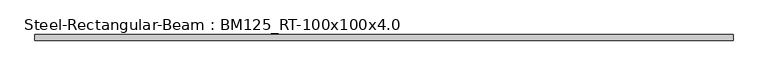
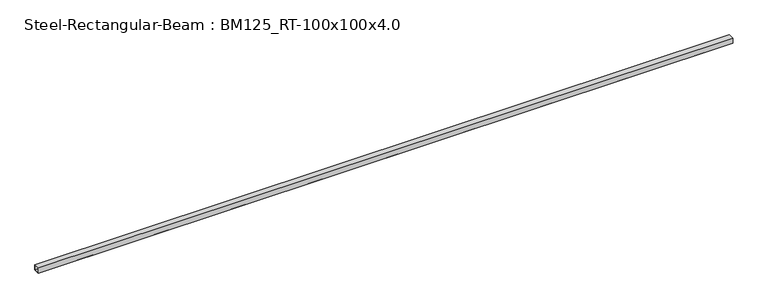
"""IFC4 building model written with IfcOpenShell, lengths in millimetres: beam geometry, Steel-Rectangular-Beam : BM125_RT-100x100x4.0."""

from ifc_helpers import new_model, si_unit, frame, origin, place, context, project, spatial, polyline, outline, extrude, source, transform, mapped, element, save


def steel_rectangular_beam_bm125_rt_100x100x4_0_88b81966(model_context):
    return source(origin(), model_context, "Body", "SweptSolid", [
        extrude(outline(polyline([(-50.0, 50.0), (50.0, 50.0), (50.0, -50.0), (-50.0, -50.0), (-50.0, 50.0)]), holes=[polyline([(46.0, -46.0), (46.0, 46.0), (-46.0, 46.0), (-46.0, -46.0), (46.0, -46.0)])]), frame((-6200.0, 0.0, 0.0), z_axis=(1.0, 0.0, 0.0), x_axis=(0.0, 1.0, 0.0)), (0.0, 0.0, 1.0), 12400.0),
        extrude(outline(polyline([(-50.0, 50.0), (50.0, 50.0), (50.0, -50.0), (-50.0, -50.0), (-50.0, 50.0)]), holes=[polyline([(46.0, -46.0), (46.0, 46.0), (-46.0, 46.0), (-46.0, -46.0), (46.0, -46.0)])]), frame((-6200.0, 0.0, 0.0), z_axis=(1.0, 0.0, 0.0), x_axis=(0.0, 1.0, 0.0)), (0.0, 0.0, 1.0), 12400.0),
        extrude(outline(polyline([(-50.0, 50.0), (50.0, 50.0), (50.0, -50.0), (-50.0, -50.0), (-50.0, 50.0)]), holes=[polyline([(46.0, -46.0), (46.0, 46.0), (-46.0, 46.0), (-46.0, -46.0), (46.0, -46.0)])]), frame((-6200.0, 0.0, 0.0), z_axis=(1.0, 0.0, 0.0), x_axis=(0.0, 1.0, 0.0)), (0.0, 0.0, 1.0), 12400.0),
        extrude(outline(polyline([(-50.0, 50.0), (50.0, 50.0), (50.0, -50.0), (-50.0, -50.0), (-50.0, 50.0)]), holes=[polyline([(46.0, -46.0), (46.0, 46.0), (-46.0, 46.0), (-46.0, -46.0), (46.0, -46.0)])]), frame((-6200.0, 0.0, 0.0), z_axis=(1.0, 0.0, 0.0), x_axis=(0.0, 1.0, 0.0)), (0.0, 0.0, 1.0), 12400.0),
    ])


if __name__ == "__main__":
    model = new_model("IFC4")
    model_context = context("Model", 3, world=origin())
    ifc_project = project(units=[si_unit("LENGTHUNIT", "METRE", prefix="MILLI")], contexts=[model_context])
    site = spatial("IfcSite", under=ifc_project)
    building = spatial("IfcBuilding", under=site)
    placement = place(None, origin())
    steel_rectangular_beam_bm125_rt_100x100x4_0_shape = steel_rectangular_beam_bm125_rt_100x100x4_0_88b81966(model_context)
    element("IfcBeam", 1, ObjectType="Steel-Rectangular-Beam : BM125_RT-100x100x4.0", at=placement, inside=building, context=model_context, shape_type="MappedRepresentation", body=[
        mapped(steel_rectangular_beam_bm125_rt_100x100x4_0_shape, transform((0.0, 0.0, 0.0), x_axis=(1.0, 0.0, 0.0), y_axis=(0.0, 1.0, 0.0), z_axis=(0.0, 0.0, 1.0))),
    ])
    save(model, "model.ifc")

# Revit data of these elements
# Type "Steel-Rectangular-Beam : BM125_RT-100x100x4.0"
#   t = 4 mm
#   Mass per Unit Length = 11.70 kg/m
#   Surface Area = 0.386 m²/m
#   Sectional Area = 14.95 cm²
#   Length [instance default] = 3000 mm
#   H = 100 mm
#   B = 100 mm
#   hec_material4 [instance default] = none
#   hec_material3 [instance default] = none
#   hec_material2 [instance default] = none
#   hec_material1 [instance default] = none
#   Structural Material [instance default] = none
# Element 1 (IfcBeam, "Steel-Rectangular-Beam : BM125_RT-100x100x4.0")
#   hec_material2 = S01AA010-00001_Main Steel Structure Fabrication Work_Shelter/Building_Steel Painting/Coating_for Non-Fireproofed Steel Surface, Surface Preparation, Primer, Second & Final Coat
#   hec_material1 = S03AA007-00001_Main Steel Structure Erection Work_Girth & Purlin
#   Structural Material = S01AA007-00001_Main Steel Structure Fabrication Work_Shelter/Building_Girth & Purlin
#   Materials on its faces: "S01AA010-00001_Main Steel Structure Fabrication Work_Shelter/Building_Steel Painting/Coating_for Non-Fireproofed Steel Surface, Surface Preparation, Primer, Second & Final Coat"
# Materials
#   "S01AA010-00001_Main Steel Structure Fabrication Work_Shelter/Building_Steel Painting/Coating_for Non-Fireproofed Steel Surface, Surface Preparation, Primer, Second & Final Coat": class "Metal", colour RGB 120 120 120, transparency 0, Description = "Paint finished steel", W00) Work Master Code = "S01AA010-00001", W01) Work Master_Lv1 = "Main Steel Structure Fabrication Work", W02) Work Master_Lv2 = "Shelter/Building", W03) Work Master_Spec.1 = "Steel Painting/Coating", W04) Work Master_Spec.2 = "for Non-Fireproofed Steel Surface, Surface Preparation, Primer, Second & Final Coat", Cost = 0
#   "S03AA007-00001_Main Steel Structure Erection Work_Girth & Purlin": class "Metal", colour RGB 120 120 120, transparency 0, Comments = "(30KG/M>Weight)", Description = "Structural steel 50ksi", W00) Work Master Code = "S03AA007-00001", W01) Work Master_Lv1 = "Main Steel Structure Erection Work", W02) Work Master_Lv2 = "Shelter/Building", W03) Work Master_Spec.1 = "Girth & Purlin", Cost = 0
#   "S01AA007-00001_Main Steel Structure Fabrication Work_Shelter/Building_Girth & Purlin": class "Metal", colour RGB 120 120 120, transparency 0, Comments = "(30KG/M>Weight)", Description = "Structural steel 50ksi", W00) Work Master Code = "S01AA007-00001", W01) Work Master_Lv1 = "Main Steel Structure Fabrication Work", W02) Work Master_Lv2 = "Shelter/Building", W03) Work Master_Spec.1 = "Girth & Purlin", Cost = 0
